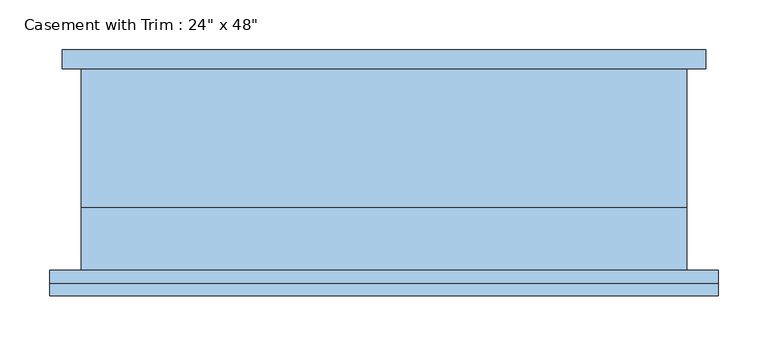
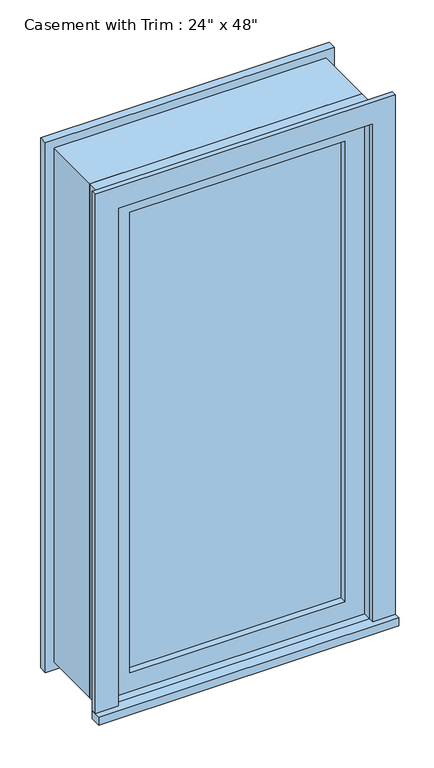
"""IFC4 building model written with IfcOpenShell, lengths in millimetres: window geometry."""

from ifc_helpers import new_model, si_unit, frame, origin, place, context, project, spatial, polyline, outline, extrude, source, transform, mapped, element, save


def window_6eb8446e(model_context):
    return source(origin(), model_context, "Body", "SweptSolid", [
        extrude(outline(polyline([(-336.55, -127.0), (-336.55, -101.6), (336.55, -101.6), (336.55, -127.0), (-336.55, -127.0)])), frame((0.0, 0.0, 914.4), z_axis=(0.0, 0.0, 1.0), x_axis=(1.0, 0.0, 0.0)), (0.0, 0.0, 1.0), 19.05),
        extrude(outline(polyline([(2114.55, -285.75), (2114.55, 285.75), (933.45, 285.75), (933.45, 336.55), (2165.35, 336.55), (2165.35, -336.55), (933.45, -336.55), (933.45, -285.75), (2114.55, -285.75)])), frame((0.0, -114.3, 0.0), z_axis=(0.0, 1.0, 0.0), x_axis=(0.0, 0.0, 1.0)), (0.0, 0.0, 1.0), 12.7),
        extrude(outline(polyline([(2152.65, 323.85), (2152.65, -323.85), (895.35, -323.85), (895.35, 323.85), (2152.65, 323.85)]), holes=[polyline([(2101.85, 273.05), (946.15, 273.05), (946.15, -273.05), (2101.85, -273.05), (2101.85, 273.05)])]), frame((0.0, 101.6, 0.0), z_axis=(0.0, 1.0, 0.0), x_axis=(0.0, 0.0, 1.0)), (0.0, 0.0, 1.0), 19.05),
        extrude(outline(polyline([(241.3, -53.975), (241.3, -66.675), (-241.3, -66.675), (-241.3, -53.975), (241.3, -53.975)])), frame((0.0, 0.0, 977.9), z_axis=(0.0, 0.0, 1.0), x_axis=(1.0, 0.0, 0.0)), (0.0, 0.0, 1.0), 1092.2),
        extrude(outline(polyline([(2114.55, -285.75), (933.45, -285.75), (933.45, 285.75), (2114.55, 285.75), (2114.55, -285.75)]), holes=[polyline([(2070.1, -241.3), (2070.1, 241.3), (977.9, 241.3), (977.9, -241.3), (2070.1, -241.3)])]), frame((0.0, -82.55, 0.0), z_axis=(0.0, 1.0, 0.0), x_axis=(0.0, 0.0, 1.0)), (0.0, 0.0, 1.0), 44.45),
        extrude(outline(polyline([(2133.6, -304.8), (914.4, -304.8), (914.4, 304.8), (2133.6, 304.8), (2133.6, -304.8)]), holes=[polyline([(2101.85, -273.05), (2101.85, 273.05), (946.15, 273.05), (946.15, -273.05), (2101.85, -273.05)])]), frame((0.0, -38.1, 0.0), z_axis=(0.0, 1.0, 0.0), x_axis=(0.0, 0.0, 1.0)), (0.0, 0.0, 1.0), 139.7),
        extrude(outline(polyline([(2133.6, 304.8), (2133.6, -304.8), (914.4, -304.8), (914.4, 304.8), (2133.6, 304.8)]), holes=[polyline([(2114.55, 285.75), (933.45, 285.75), (933.45, -285.75), (2114.55, -285.75), (2114.55, 285.75)])]), frame((0.0, -101.6, 0.0), z_axis=(0.0, 1.0, 0.0), x_axis=(0.0, 0.0, 1.0)), (0.0, 0.0, 1.0), 63.5),
    ])


if __name__ == "__main__":
    model = new_model("IFC4")
    model_context = context("Model", 3, world=origin())
    ifc_project = project(units=[si_unit("LENGTHUNIT", "METRE", prefix="MILLI")], contexts=[model_context])
    site = spatial("IfcSite", under=ifc_project)
    building = spatial("IfcBuilding", under=site)
    placement = place(None, origin())
    window_shape = window_6eb8446e(model_context)
    element("IfcWindow", 1, ObjectType="Casement with Trim : 24\" x 48\"", at=placement, inside=building, context=model_context, shape_type="MappedRepresentation", body=[
        mapped(window_shape, transform((0.0, 0.0, 0.0), x_axis=(1.0, 0.0, 0.0), y_axis=(0.0, 1.0, 0.0), z_axis=(0.0, 0.0, 1.0))),
    ])
    save(model, "model.ifc")

# Revit data of these elements
# Type "Casement with Trim : 24\" x 48\""
#   Type Mark = "39"
#   Assembly Code = "B2020100"
#   Height = 4' - 0"
#   Default Sill Height = 3' - 0"
#   Trim Projection - Ext. = 0' - 0 1/2"
#   Trim Projection - Int. = 0' - 0 3/4"
#   Trim Width - Exterior = 0' - 2"
#   Trim Width - Interior = 0' - 2"
#   Width = 2' - 0"
#   Window Inset = 0' - 0 3/4"
#   Glass Pane Material = Glass
#   Sash Material = Sash
#   Trim Exterior Material = Trim
#   Trim Interior Material = Trim
#   Wall Closure = (empty or 0)
# Element 1 (IfcWindow, "Casement with Trim : 24\" x 48\"")
#   Materials on its faces: "Sash", "Trim", "Glass"
# Materials
#   "Glass": class "Glass", colour RGB 0 128 192, transparency 0.75
#   "Sash": class "Wood", colour RGB 224 178 126, transparency 0
#   "Trim": class "Wood", colour RGB 224 178 126, transparency 0
